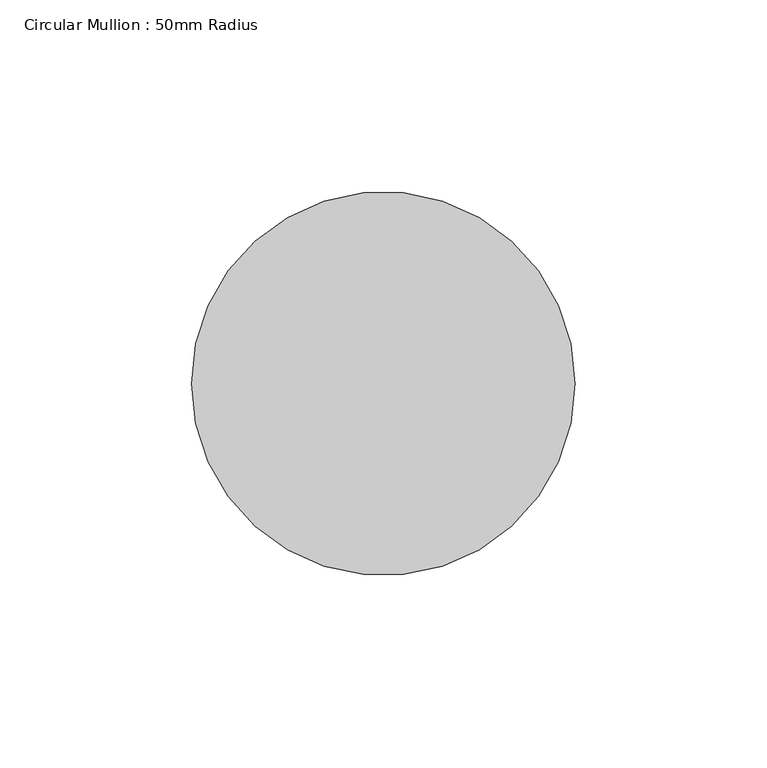
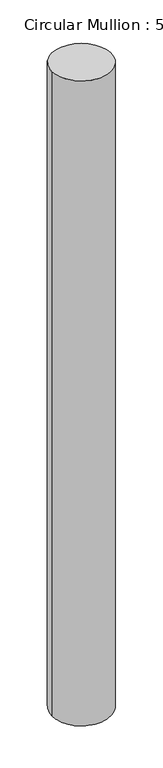
"""IFC4 building model written with IfcOpenShell, lengths in millimetres: member geometry, Circular Mullion : 50mm Radius."""

from ifc_helpers import new_model, si_unit, frame, origin, place, context, project, spatial, ellipse_curve, source, transform, mapped, element, save
from ifc_brep_helpers import plane_surface, cylinder_surface, advanced_brep


def circular_mullion_50mm_radius_ad5664ad(model_context):
    return source(origin(), model_context, "Body", "AdvancedBrep", [
        advanced_brep(
        [(-100.0, 0.0, 1.4680128), (0.0, 0.0, 0.0), (0.0, 0.0, -1152.6744857), (-100.0, 0.0, -1154.0655863)],
        [
            (0, 1, ellipse_curve(frame((-50.0, 0.0, 0.7340064), z_axis=(-0.014675464026278739, -0.020493332759839673, -0.9996822765599118), x_axis=(-0.5820344729133072, -0.8127733548834735, 0.025206069348311065)), 50.0158912, 50.0)),
            (1, 2),
            (2, 3, ellipse_curve(frame((-50.0, 0.0, -1153.370036), z_axis=(-0.013907037053686778, -0.01942027438003122, 0.9997146829287804), x_axis=(0.5820533405318324, 0.8127997022877941, 0.02388624576210974)), 50.0142699, 50.0)),
            (3, 0),
            (1, 0, ellipse_curve(frame((-50.0, 0.0, 0.7340064), z_axis=(-0.014675464026278739, -0.020493332759839673, -0.9996822765599118), x_axis=(-0.5820344729133072, -0.8127733548834735, 0.025206069348311065)), 50.0158912, 50.0)),
            (3, 2, ellipse_curve(frame((-50.0, 0.0, -1153.370036), z_axis=(-0.013907037053686778, -0.01942027438003122, 0.9997146829287804), x_axis=(0.5820533405318324, 0.8127997022877941, 0.02388624576210974)), 50.0142699, 50.0)),
        ],
        [
            cylinder_surface(frame((-50.0, 0.0, 0.0), z_axis=(0.0, 0.0, 1.0), x_axis=(1.0, 0.0, 0.0)), 50.0),
            plane_surface(frame((-247.8120543, 177.4604907, 0.0), z_axis=(0.014675464026278739, 0.020493332759839673, 0.9996822765599118), x_axis=(0.582034472913305, 0.8127733548834749, -0.02520606934831608))),
            plane_surface(frame((-247.8120543, 177.4604907, -1152.6744857), z_axis=(0.013907037053686778, 0.01942027438003122, -0.9997146829287804), x_axis=(0.5820533405318324, 0.812799702287794, 0.02388624576211829))),
        ],
        [
            (0, [[1, 2, 3, 4]]),
            (0, [[5, -4, 6, -2]]),
            (1, [[-1, -5]]),
            (2, [[-6, -3]]),
        ],
    ),
    ])


if __name__ == "__main__":
    model = new_model("IFC4")
    model_context = context("Model", 3, world=origin())
    ifc_project = project(units=[si_unit("LENGTHUNIT", "METRE", prefix="MILLI")], contexts=[model_context])
    site = spatial("IfcSite", under=ifc_project)
    building = spatial("IfcBuilding", under=site)
    placement = place(None, origin())
    circular_mullion_50mm_radius_shape = circular_mullion_50mm_radius_ad5664ad(model_context)
    element("IfcMember", 1, ObjectType="Circular Mullion : 50mm Radius", at=placement, inside=building, context=model_context, shape_type="MappedRepresentation", body=[
        mapped(circular_mullion_50mm_radius_shape, transform((0.0, 0.0, 0.0), x_axis=(1.0, 0.0, 0.0), y_axis=(0.0, 1.0, 0.0), z_axis=(0.0, 0.0, 1.0))),
    ])
    save(model, "model.ifc")

# Revit data of these elements
# Type "Circular Mullion : 50mm Radius"
#   built-in parameter 1007350 = 0.164042 (stored number, unit not read)
# Element 1 (IfcMember, "Circular Mullion : 50mm Radius")
#   Materials on its faces: "Aluminium"
# Materials
#   "Aluminium": class "Metal", colour RGB 247 247 247, transparency 0, Description = "Aluminium 6061", Cost = 0
